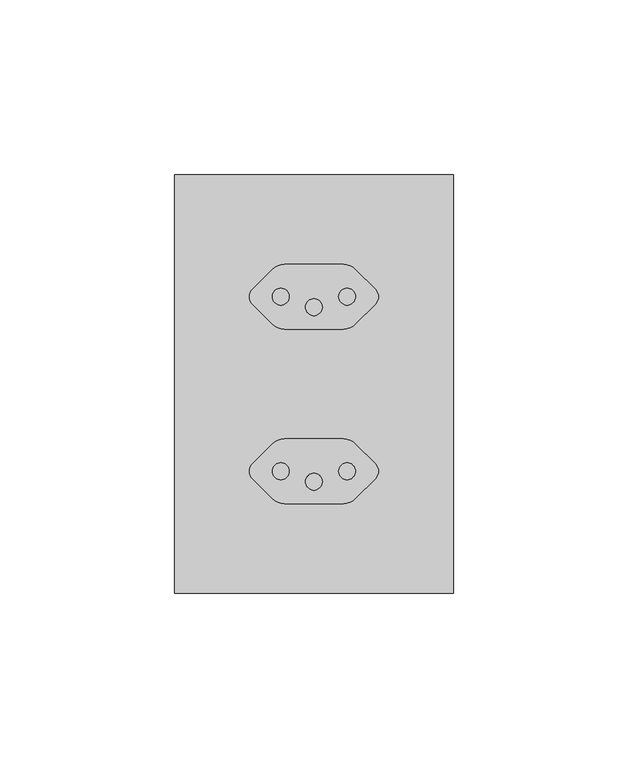
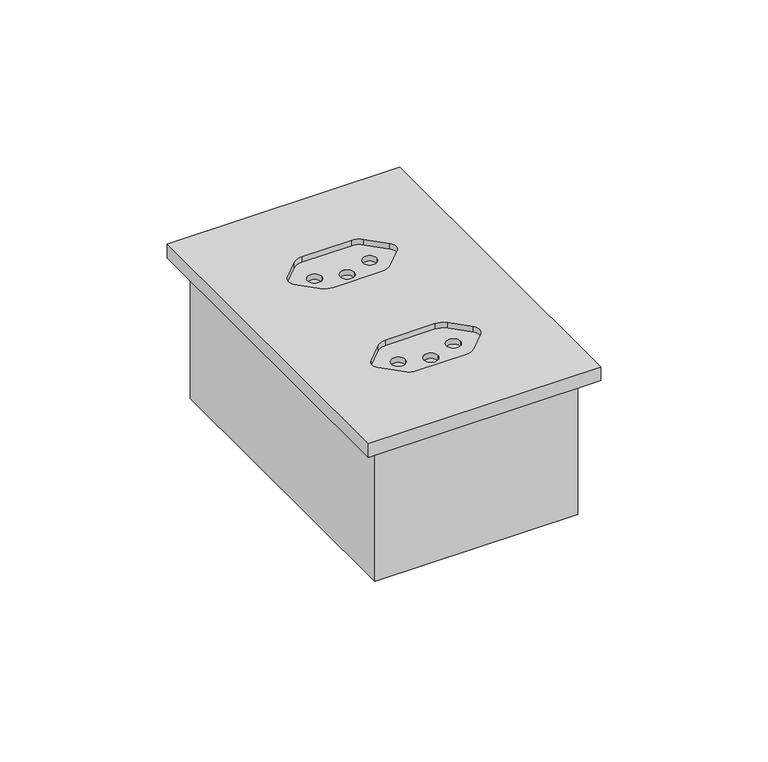
"""IFC4 building model written with IfcOpenShell, lengths in millimetres: proxy geometry, CAIXA VERTICE V7 : Tomada 20A 2s."""

from ifc_helpers import new_model, si_unit, frame, origin, place, context, project, spatial, polyline, circle_curve, faceted_brep, source, transform, mapped, element, save
from ifc_brep_helpers import plane_surface, revolved_surface, advanced_brep


def electrical_fixtures_6b1fb481(model_context):
    return source(origin(), model_context, "Body", "SolidModel", [
        faceted_brep([(33.0, -947.0, -48.0), (-33.0, -947.0, -48.0), (-33.0, -1053.0, -48.0), (33.0, -1053.0, -48.0), (35.0, -1055.0, -50.0), (-35.0, -1055.0, -50.0), (-35.0, -945.0, -50.0), (35.0, -945.0, -50.0), (35.0, -1055.0, 0.0), (-35.0, -1055.0, 0.0), (-35.0, -945.0, 0.0), (35.0, -945.0, 0.0), (33.0, -1053.0, 0.0), (-33.0, -1053.0, 0.0), (-33.0, -947.0, 0.0), (33.0, -947.0, 0.0)], [[[0, 1, 2, 3]], [[4, 5, 6, 7]], [[4, 8, 9, 5]], [[9, 10, 6, 5]], [[10, 11, 7, 6]], [[11, 8, 4, 7]], [[8, 11, 10, 9], [12, 13, 14, 15]], [[15, 0, 3, 12]], [[14, 1, 0, 15]], [[13, 2, 1, 14]], [[12, 3, 2, 13]]]),
        advanced_brep(
        [(40.0, -1060.0, 5.0), (40.0, -940.0, 5.0), (-40.0, -940.0, 5.0), (-40.0, -1060.0, 5.0), (8.4215729, -1015.75, 5.0), (11.9571068, -1017.2144661, 5.0), (17.6213203, -1022.8786797, 5.0), (17.6213203, -1027.1213203, 5.0), (11.9571068, -1032.7855339, 5.0), (8.4215729, -1034.25, 5.0), (-8.4215729, -1034.25, 5.0), (-11.9571068, -1032.7855339, 5.0), (-17.6213203, -1027.1213203, 5.0), (-17.6213203, -1022.8786797, 5.0), (-11.9571068, -1017.2144661, 5.0), (-8.4215729, -1015.75, 5.0), (8.4215729, -965.75, 5.0), (11.9571068, -967.2144661, 5.0), (17.6213203, -972.8786797, 5.0), (17.6213203, -977.1213203, 5.0), (11.9571068, -982.7855339, 5.0), (8.4215729, -984.25, 5.0), (-8.4215729, -984.25, 5.0), (-11.9571068, -982.7855339, 5.0), (-17.6213203, -977.1213203, 5.0), (-17.6213203, -972.8786797, 5.0), (-11.9571068, -967.2144661, 5.0), (-8.4215729, -965.75, 5.0), (-40.0, -1060.0, 0.0), (-40.0, -940.0, 0.0), (40.0, -940.0, 0.0), (40.0, -1060.0, 0.0), (8.4215729, -1015.75, 3.0), (-8.4215729, -1015.75, 3.0), (-11.9571068, -1017.2144661, 3.0), (-17.6213203, -1022.8786797, 3.0), (-17.6213203, -1027.1213203, 3.0), (-11.9571068, -1032.7855339, 3.0), (-8.4215729, -1034.25, 3.0), (8.4215729, -1034.25, 3.0), (11.9571068, -1032.7855339, 3.0), (17.6213203, -1027.1213203, 3.0), (17.6213203, -1022.8786797, 3.0), (11.9571068, -1017.2144661, 3.0), (-7.1, -1025.0, 3.0), (-11.9, -1025.0, 3.0), (11.9, -1025.0, 3.0), (7.1, -1025.0, 3.0), (2.4, -1028.0, 3.0), (-2.4, -1028.0, 3.0), (-11.9, -1025.0, 1.0), (-7.1, -1025.0, 1.0), (7.1, -1025.0, 1.0), (11.9, -1025.0, 1.0), (-2.4, -1028.0, 1.0), (2.4, -1028.0, 1.0), (8.4215729, -965.75, 3.0), (-8.4215729, -965.75, 3.0), (-11.9571068, -967.2144661, 3.0), (-17.6213203, -972.8786797, 3.0), (-17.6213203, -977.1213203, 3.0), (-11.9571068, -982.7855339, 3.0), (-8.4215729, -984.25, 3.0), (8.4215729, -984.25, 3.0), (11.9571068, -982.7855339, 3.0), (17.6213203, -977.1213203, 3.0), (17.6213203, -972.8786797, 3.0), (11.9571068, -967.2144661, 3.0), (-7.1, -975.0, 3.0), (-11.9, -975.0, 3.0), (11.9, -975.0, 3.0), (7.1, -975.0, 3.0), (2.4, -978.0, 3.0), (-2.4, -978.0, 3.0), (-11.9, -975.0, 1.0), (-7.1, -975.0, 1.0), (7.1, -975.0, 1.0), (11.9, -975.0, 1.0), (-2.4, -978.0, 1.0), (2.4, -978.0, 1.0)],
        [
            (0, 1),
            (1, 2),
            (2, 3),
            (3, 0),
            (4, 5, circle_curve(frame((8.4215729, -1020.75, 5.0), z_axis=(0.0, 0.0, -1.0), x_axis=(-1.0, 0.0, 0.0)), 5.0)),
            (5, 6),
            (6, 7, circle_curve(frame((15.5, -1025.0, 5.0), z_axis=(0.0, 0.0, -1.0), x_axis=(-1.0, 0.0, 0.0)), 3.0)),
            (7, 8),
            (8, 9, circle_curve(frame((8.4215729, -1029.25, 5.0), z_axis=(0.0, 0.0, -1.0), x_axis=(-1.0, 0.0, 0.0)), 5.0)),
            (9, 10),
            (10, 11, circle_curve(frame((-8.4215729, -1029.25, 5.0), z_axis=(0.0, 0.0, -1.0), x_axis=(-1.0, 0.0, 0.0)), 5.0)),
            (11, 12),
            (12, 13, circle_curve(frame((-15.5, -1025.0, 5.0), z_axis=(0.0, 0.0, -1.0), x_axis=(-1.0, 0.0, 0.0)), 3.0)),
            (13, 14),
            (14, 15, circle_curve(frame((-8.4215729, -1020.75, 5.0), z_axis=(0.0, 0.0, -1.0), x_axis=(-1.0, 0.0, 0.0)), 5.0)),
            (15, 4),
            (16, 17, circle_curve(frame((8.4215729, -970.75, 5.0), z_axis=(0.0, 0.0, -1.0), x_axis=(-1.0, 0.0, 0.0)), 5.0)),
            (17, 18),
            (18, 19, circle_curve(frame((15.5, -975.0, 5.0), z_axis=(0.0, 0.0, -1.0), x_axis=(-1.0, 0.0, 0.0)), 3.0)),
            (19, 20),
            (20, 21, circle_curve(frame((8.4215729, -979.25, 5.0), z_axis=(0.0, 0.0, -1.0), x_axis=(-1.0, 0.0, 0.0)), 5.0)),
            (21, 22),
            (22, 23, circle_curve(frame((-8.4215729, -979.25, 5.0), z_axis=(0.0, 0.0, -1.0), x_axis=(-1.0, 0.0, 0.0)), 5.0)),
            (23, 24),
            (24, 25, circle_curve(frame((-15.5, -975.0, 5.0), z_axis=(0.0, 0.0, -1.0), x_axis=(-1.0, 0.0, 0.0)), 3.0)),
            (25, 26),
            (26, 27, circle_curve(frame((-8.4215729, -970.75, 5.0), z_axis=(0.0, 0.0, -1.0), x_axis=(-1.0, 0.0, 0.0)), 5.0)),
            (27, 16),
            (28, 29),
            (29, 30),
            (30, 31),
            (31, 28),
            (3, 28),
            (31, 0),
            (2, 29),
            (1, 30),
            (32, 33),
            (33, 34, circle_curve(frame((-8.4215729, -1020.75, 3.0), z_axis=(0.0, 0.0, 1.0), x_axis=(-1.0, 0.0, 0.0)), 5.0)),
            (34, 35),
            (35, 36, circle_curve(frame((-15.5, -1025.0, 3.0), z_axis=(0.0, 0.0, 1.0), x_axis=(-1.0, 0.0, 0.0)), 3.0)),
            (36, 37),
            (37, 38, circle_curve(frame((-8.4215729, -1029.25, 3.0), z_axis=(0.0, 0.0, 1.0), x_axis=(-1.0, 0.0, 0.0)), 5.0)),
            (38, 39),
            (39, 40, circle_curve(frame((8.4215729, -1029.25, 3.0), z_axis=(0.0, 0.0, 1.0), x_axis=(-1.0, 0.0, 0.0)), 5.0)),
            (40, 41),
            (41, 42, circle_curve(frame((15.5, -1025.0, 3.0), z_axis=(0.0, 0.0, 1.0), x_axis=(-1.0, 0.0, 0.0)), 3.0)),
            (42, 43),
            (43, 32, circle_curve(frame((8.4215729, -1020.75, 3.0), z_axis=(0.0, 0.0, 1.0), x_axis=(-1.0, 0.0, 0.0)), 5.0)),
            (44, 45, circle_curve(frame((-9.5, -1025.0, 3.0), z_axis=(0.0, 0.0, -1.0), x_axis=(1.0, -2.301812013077709e-12, 0.0)), 2.4)),
            (45, 44, circle_curve(frame((-9.5, -1025.0, 3.0), z_axis=(0.0, 0.0, -1.0), x_axis=(1.0, -2.301812013077709e-12, 0.0)), 2.4)),
            (46, 47, circle_curve(frame((9.5, -1025.0, 3.0), z_axis=(0.0, 0.0, -1.0), x_axis=(1.0, -2.301812013077709e-12, 0.0)), 2.4)),
            (47, 46, circle_curve(frame((9.5, -1025.0, 3.0), z_axis=(0.0, 0.0, -1.0), x_axis=(1.0, -2.301812013077709e-12, 0.0)), 2.4)),
            (48, 49, circle_curve(frame((0.0, -1028.0, 3.0), z_axis=(0.0, 0.0, -1.0), x_axis=(1.0, -2.301812013077709e-12, 0.0)), 2.4)),
            (49, 48, circle_curve(frame((0.0, -1028.0, 3.0), z_axis=(0.0, 0.0, -1.0), x_axis=(1.0, -2.301812013077709e-12, 0.0)), 2.4)),
            (32, 4),
            (15, 33),
            (14, 34),
            (13, 35),
            (12, 36),
            (11, 37),
            (10, 38),
            (9, 39),
            (8, 40),
            (7, 41),
            (6, 42),
            (5, 43),
            (50, 51, circle_curve(frame((-9.5, -1025.0, 1.0), z_axis=(0.0, 0.0, 1.0), x_axis=(1.0, -2.301812013077709e-12, 0.0)), 2.4)),
            (51, 50, circle_curve(frame((-9.5, -1025.0, 1.0), z_axis=(0.0, 0.0, 1.0), x_axis=(1.0, -2.301812013077709e-12, 0.0)), 2.4)),
            (52, 53, circle_curve(frame((9.5, -1025.0, 1.0), z_axis=(0.0, 0.0, 1.0), x_axis=(1.0, -2.301812013077709e-12, 0.0)), 2.4)),
            (53, 52, circle_curve(frame((9.5, -1025.0, 1.0), z_axis=(0.0, 0.0, 1.0), x_axis=(1.0, -2.301812013077709e-12, 0.0)), 2.4)),
            (54, 55, circle_curve(frame((0.0, -1028.0, 1.0), z_axis=(0.0, 0.0, 1.0), x_axis=(1.0, -2.301812013077709e-12, 0.0)), 2.4)),
            (55, 54, circle_curve(frame((0.0, -1028.0, 1.0), z_axis=(0.0, 0.0, 1.0), x_axis=(1.0, -2.301812013077709e-12, 0.0)), 2.4)),
            (45, 50),
            (51, 44),
            (47, 52),
            (53, 46),
            (49, 54),
            (55, 48),
            (56, 57),
            (57, 58, circle_curve(frame((-8.4215729, -970.75, 3.0), z_axis=(0.0, 0.0, 1.0), x_axis=(-1.0, 0.0, 0.0)), 5.0)),
            (58, 59),
            (59, 60, circle_curve(frame((-15.5, -975.0, 3.0), z_axis=(0.0, 0.0, 1.0), x_axis=(-1.0, 0.0, 0.0)), 3.0)),
            (60, 61),
            (61, 62, circle_curve(frame((-8.4215729, -979.25, 3.0), z_axis=(0.0, 0.0, 1.0), x_axis=(-1.0, 0.0, 0.0)), 5.0)),
            (62, 63),
            (63, 64, circle_curve(frame((8.4215729, -979.25, 3.0), z_axis=(0.0, 0.0, 1.0), x_axis=(-1.0, 0.0, 0.0)), 5.0)),
            (64, 65),
            (65, 66, circle_curve(frame((15.5, -975.0, 3.0), z_axis=(0.0, 0.0, 1.0), x_axis=(-1.0, 0.0, 0.0)), 3.0)),
            (66, 67),
            (67, 56, circle_curve(frame((8.4215729, -970.75, 3.0), z_axis=(0.0, 0.0, 1.0), x_axis=(-1.0, 0.0, 0.0)), 5.0)),
            (68, 69, circle_curve(frame((-9.5, -975.0, 3.0), z_axis=(0.0, 0.0, -1.0), x_axis=(1.0, -2.301812013077709e-12, 0.0)), 2.4)),
            (69, 68, circle_curve(frame((-9.5, -975.0, 3.0), z_axis=(0.0, 0.0, -1.0), x_axis=(1.0, -2.301812013077709e-12, 0.0)), 2.4)),
            (70, 71, circle_curve(frame((9.5, -975.0, 3.0), z_axis=(0.0, 0.0, -1.0), x_axis=(1.0, -2.301812013077709e-12, 0.0)), 2.4)),
            (71, 70, circle_curve(frame((9.5, -975.0, 3.0), z_axis=(0.0, 0.0, -1.0), x_axis=(1.0, -2.301812013077709e-12, 0.0)), 2.4)),
            (72, 73, circle_curve(frame((0.0, -978.0, 3.0), z_axis=(0.0, 0.0, -1.0), x_axis=(1.0, -2.301812013077709e-12, 0.0)), 2.4)),
            (73, 72, circle_curve(frame((0.0, -978.0, 3.0), z_axis=(0.0, 0.0, -1.0), x_axis=(1.0, -2.301812013077709e-12, 0.0)), 2.4)),
            (56, 16),
            (27, 57),
            (26, 58),
            (25, 59),
            (24, 60),
            (23, 61),
            (22, 62),
            (21, 63),
            (20, 64),
            (19, 65),
            (18, 66),
            (17, 67),
            (74, 75, circle_curve(frame((-9.5, -975.0, 1.0), z_axis=(0.0, 0.0, 1.0), x_axis=(1.0, -2.301812013077709e-12, 0.0)), 2.4)),
            (75, 74, circle_curve(frame((-9.5, -975.0, 1.0), z_axis=(0.0, 0.0, 1.0), x_axis=(1.0, -2.301812013077709e-12, 0.0)), 2.4)),
            (76, 77, circle_curve(frame((9.5, -975.0, 1.0), z_axis=(0.0, 0.0, 1.0), x_axis=(1.0, -2.301812013077709e-12, 0.0)), 2.4)),
            (77, 76, circle_curve(frame((9.5, -975.0, 1.0), z_axis=(0.0, 0.0, 1.0), x_axis=(1.0, -2.301812013077709e-12, 0.0)), 2.4)),
            (78, 79, circle_curve(frame((0.0, -978.0, 1.0), z_axis=(0.0, 0.0, 1.0), x_axis=(1.0, -2.301812013077709e-12, 0.0)), 2.4)),
            (79, 78, circle_curve(frame((0.0, -978.0, 1.0), z_axis=(0.0, 0.0, 1.0), x_axis=(1.0, -2.301812013077709e-12, 0.0)), 2.4)),
            (69, 74),
            (75, 68),
            (71, 76),
            (77, 70),
            (73, 78),
            (79, 72),
        ],
        [
            plane_surface(frame((-60.0, -1060.0, 5.0), z_axis=(0.0, 0.0, 1.0), x_axis=(-1.0, 0.0, 0.0))),
            plane_surface(frame((-60.0, -1060.0, 0.0), z_axis=(0.0, 0.0, -1.0), x_axis=(1.0, 0.0, 0.0))),
            plane_surface(frame((40.0, -1060.0, 5.0), z_axis=(0.0, -1.0, 0.0), x_axis=(0.0, 0.0, -1.0))),
            plane_surface(frame((-40.0, -1060.0, 5.0), z_axis=(-1.0, 0.0, 0.0), x_axis=(0.0, 0.0, -1.0))),
            plane_surface(frame((-40.0, -940.0, 5.0), z_axis=(0.0, 1.0, 0.0), x_axis=(0.0, 0.0, -1.0))),
            plane_surface(frame((40.0, -940.0, 5.0), z_axis=(1.0, 0.0, 0.0), x_axis=(0.0, 0.0, -1.0))),
            plane_surface(frame((3.4215729, -1020.75, 3.0), z_axis=(0.0, 0.0, 1.0), x_axis=(0.0, -1.0, 0.0))),
            plane_surface(frame((-8.4215729, -1015.75, 5.0), z_axis=(0.0, -1.0, 0.0), x_axis=(0.0, 0.0, -1.0))),
            revolved_surface(polyline([(-13.4215729, -1020.75, 5.0), (-13.4215729, -1020.75, 3.0)]), (-8.4215729, -1020.75, 3.0), (0.0, 0.0, 1.0)),
            plane_surface(frame((-17.6213203, -1022.8786797, 5.0), z_axis=(0.7071067811865045, -0.7071067811865905, 0.0), x_axis=(0.0, 0.0, -1.0))),
            revolved_surface(polyline([(-18.5, -1025.0, 5.0), (-18.5, -1025.0, 3.0)]), (-15.5, -1025.0, 3.0), (0.0, 0.0, 1.0)),
            plane_surface(frame((-11.9571068, -1032.7855339, 5.0), z_axis=(0.7071067811865515, 0.7071067811865437, 0.0), x_axis=(0.0, 0.0, -1.0))),
            revolved_surface(polyline([(-13.4215729, -1029.25, 5.0), (-13.4215729, -1029.25, 3.0)]), (-8.4215729, -1029.25, 3.0), (0.0, 0.0, 1.0)),
            plane_surface(frame((8.4215729, -1034.25, 5.0), z_axis=(0.0, 1.0, 0.0), x_axis=(0.0, 0.0, -1.0))),
            revolved_surface(polyline([(3.4215728999999993, -1029.25, 5.0), (3.4215728999999993, -1029.25, 3.0)]), (8.4215729, -1029.25, 3.0), (0.0, 0.0, 1.0)),
            plane_surface(frame((17.6213203, -1027.1213203, 5.0), z_axis=(-0.7071067811865307, 0.7071067811865643, 0.0), x_axis=(0.0, 0.0, -1.0))),
            revolved_surface(polyline([(12.5, -1025.0, 5.0), (12.5, -1025.0, 3.0)]), (15.5, -1025.0, 3.0), (0.0, 0.0, 1.0)),
            plane_surface(frame((11.9571068, -1017.2144661, 5.0), z_axis=(-0.7071067811865893, -0.7071067811865058, 0.0), x_axis=(0.0, 0.0, -1.0))),
            revolved_surface(polyline([(3.4215728999999993, -1020.75, 5.0), (3.4215728999999993, -1020.75, 3.0)]), (8.4215729, -1020.75, 3.0), (0.0, 0.0, 1.0)),
            plane_surface(frame((-7.1, -1025.0, 1.0), z_axis=(0.0, 0.0, 1.0), x_axis=(2.301812013077709e-12, 1.0, 0.0))),
            revolved_surface(polyline([(-7.1, -1025.0000000000055, 3.0), (-7.1, -1025.0000000000055, 1.0)]), (-9.5, -1025.0, 1.0), (0.0, 0.0, 1.0)),
            revolved_surface(polyline([(11.9, -1025.0000000000055, 3.0), (11.9, -1025.0000000000055, 1.0)]), (9.5, -1025.0, 5.0), (0.0, 0.0, 1.0)),
            revolved_surface(polyline([(2.4, -1028.0000000000055, 3.0), (2.4, -1028.0000000000055, 1.0)]), (0.0, -1028.0, 5.0), (0.0, 0.0, 1.0)),
            plane_surface(frame((3.4215729, -970.75, 3.0), z_axis=(0.0, 0.0, 1.0), x_axis=(0.0, -1.0, 0.0))),
            plane_surface(frame((-8.4215729, -965.75, 5.0), z_axis=(0.0, -1.0, 0.0), x_axis=(0.0, 0.0, -1.0))),
            revolved_surface(polyline([(-13.4215729, -970.75, 5.0), (-13.4215729, -970.75, 3.0)]), (-8.4215729, -970.75, 3.0), (0.0, 0.0, 1.0)),
            plane_surface(frame((-17.6213203, -972.8786797, 5.0), z_axis=(0.7071067811865045, -0.7071067811865905, 0.0), x_axis=(0.0, 0.0, -1.0))),
            revolved_surface(polyline([(-18.5, -975.0, 5.0), (-18.5, -975.0, 3.0)]), (-15.5, -975.0, 3.0), (0.0, 0.0, 1.0)),
            plane_surface(frame((-11.9571068, -982.7855339, 5.0), z_axis=(0.7071067811865515, 0.7071067811865437, 0.0), x_axis=(0.0, 0.0, -1.0))),
            revolved_surface(polyline([(-13.4215729, -979.25, 5.0), (-13.4215729, -979.25, 3.0)]), (-8.4215729, -979.25, 3.0), (0.0, 0.0, 1.0)),
            plane_surface(frame((8.4215729, -984.25, 5.0), z_axis=(0.0, 1.0, 0.0), x_axis=(0.0, 0.0, -1.0))),
            revolved_surface(polyline([(3.4215728999999993, -979.25, 5.0), (3.4215728999999993, -979.25, 3.0)]), (8.4215729, -979.25, 3.0), (0.0, 0.0, 1.0)),
            plane_surface(frame((17.6213203, -977.1213203, 5.0), z_axis=(-0.7071067811865307, 0.7071067811865643, 0.0), x_axis=(0.0, 0.0, -1.0))),
            revolved_surface(polyline([(12.5, -975.0, 5.0), (12.5, -975.0, 3.0)]), (15.5, -975.0, 3.0), (0.0, 0.0, 1.0)),
            plane_surface(frame((11.9571068, -967.2144661, 5.0), z_axis=(-0.7071067811865893, -0.7071067811865058, 0.0), x_axis=(0.0, 0.0, -1.0))),
            revolved_surface(polyline([(3.4215728999999993, -970.75, 5.0), (3.4215728999999993, -970.75, 3.0)]), (8.4215729, -970.75, 3.0), (0.0, 0.0, 1.0)),
            plane_surface(frame((-7.1, -975.0, 1.0), z_axis=(0.0, 0.0, 1.0), x_axis=(2.301812013077709e-12, 1.0, 0.0))),
            revolved_surface(polyline([(-7.1, -975.0000000000056, 3.0), (-7.1, -975.0000000000056, 1.0)]), (-9.5, -975.0, 1.0), (0.0, 0.0, 1.0)),
            revolved_surface(polyline([(11.9, -975.0000000000056, 3.0), (11.9, -975.0000000000056, 1.0)]), (9.5, -975.0, 5.0), (0.0, 0.0, 1.0)),
            revolved_surface(polyline([(2.4, -978.0000000000056, 3.0), (2.4, -978.0000000000056, 1.0)]), (0.0, -978.0, 5.0), (0.0, 0.0, 1.0)),
        ],
        [
            (0, [[1, 2, 3, 4], [5, 6, 7, 8, 9, 10, 11, 12, 13, 14, 15, 16], [17, 18, 19, 20, 21, 22, 23, 24, 25, 26, 27, 28]]),
            (1, [[29, 30, 31, 32]]),
            (2, [[33, -32, 34, -4]]),
            (3, [[35, -29, -33, -3]]),
            (4, [[36, -30, -35, -2]]),
            (5, [[-34, -31, -36, -1]]),
            (6, [[37, 38, 39, 40, 41, 42, 43, 44, 45, 46, 47, 48], [49, 50], [51, 52], [53, 54]]),
            (7, [[55, -16, 56, -37]]),
            (8, [[-56, -15, 57, -38]]),
            (9, [[-57, -14, 58, -39]]),
            (10, [[-58, -13, 59, -40]]),
            (11, [[-59, -12, 60, -41]]),
            (12, [[-60, -11, 61, -42]]),
            (13, [[-61, -10, 62, -43]]),
            (14, [[-62, -9, 63, -44]]),
            (15, [[-63, -8, 64, -45]]),
            (16, [[-64, -7, 65, -46]]),
            (17, [[-65, -6, 66, -47]]),
            (18, [[-66, -5, -55, -48]]),
            (19, [[67, 68]]),
            (19, [[69, 70]]),
            (19, [[71, 72]]),
            (20, [[73, -68, 74, -50]]),
            (20, [[-74, -67, -73, -49]]),
            (21, [[75, -70, 76, -52]]),
            (21, [[-76, -69, -75, -51]]),
            (22, [[77, -72, 78, -54]]),
            (22, [[-78, -71, -77, -53]]),
            (23, [[79, 80, 81, 82, 83, 84, 85, 86, 87, 88, 89, 90], [91, 92], [93, 94], [95, 96]]),
            (24, [[97, -28, 98, -79]]),
            (25, [[-98, -27, 99, -80]]),
            (26, [[-99, -26, 100, -81]]),
            (27, [[-100, -25, 101, -82]]),
            (28, [[-101, -24, 102, -83]]),
            (29, [[-102, -23, 103, -84]]),
            (30, [[-103, -22, 104, -85]]),
            (31, [[-104, -21, 105, -86]]),
            (32, [[-105, -20, 106, -87]]),
            (33, [[-106, -19, 107, -88]]),
            (34, [[-107, -18, 108, -89]]),
            (35, [[-108, -17, -97, -90]]),
            (36, [[109, 110]]),
            (36, [[111, 112]]),
            (36, [[113, 114]]),
            (37, [[115, -110, 116, -92]]),
            (37, [[-116, -109, -115, -91]]),
            (38, [[117, -112, 118, -94]]),
            (38, [[-118, -111, -117, -93]]),
            (39, [[119, -114, 120, -96]]),
            (39, [[-120, -113, -119, -95]]),
        ],
    ),
    ])


if __name__ == "__main__":
    model = new_model("IFC4")
    model_context = context("Model", 3, world=origin())
    ifc_project = project(units=[si_unit("LENGTHUNIT", "METRE", prefix="MILLI")], contexts=[model_context])
    site = spatial("IfcSite", under=ifc_project)
    building = spatial("IfcBuilding", under=site)
    placement = place(None, origin())
    electrical_fixtures_shape = electrical_fixtures_6b1fb481(model_context)
    element("IfcBuildingElementProxy", 1, Name="CAIXA VERTICE V7 : Tomada 20A 2s", ObjectType="CAIXA VERTICE V7 : Tomada 20A 2s", at=placement, inside=building, context=model_context, shape_type="MappedRepresentation", body=[
        mapped(electrical_fixtures_shape, transform((0.0, 0.0, 0.0), x_axis=(1.0, 0.0, 0.0), y_axis=(0.0, 1.0, 0.0), z_axis=(0.0, 0.0, 1.0))),
    ])
    save(model, "model.ifc")

# Revit data of these elements
# Type "CAIXA VERTICE V7 : Tomada 20A 2s"
#   URL = "www.facebook.com/verticetreinamentos"
#   SEÇÃO [instance default] = ""
#   Rotação [instance default] = 0.00°
#   LARGURA DA TAMPA = 0.08 m
#   BORDA = 0.01 m
#   ALTURA DE INSTALAÇÃO [instance default] = 1.10 m
#   Distância Anotação [instance default] = 0.0015 m
#   ALTURA DA TAMPA = 0.12 m
#   Vertical [instance default] = yes
#   VER SEÇÃO [instance default] = no
#   SHADE ESQ [instance default] = no
#   SHADE DIR [instance default] = yes
#   HORIZONTAL [instance default] = no
#   ANDAR COM A LEGENDA [instance default] = 0
#   Material Tampa [instance default] = Plástico, branco opaco
#   Caixa = element 1798518
#   Anotação = element 1798532
#   Default Elevation = 0
# Element 1 (IfcBuildingElementProxy, "CAIXA VERTICE V7 : Tomada 20A 2s")
#   ALTURA DE INSTALAÇÃO = 1.00 m
#   Materials on its faces: "Plástico, branco opaco"
# Materials
#   "Plástico, branco opaco": class "Plástico", colour RGB 120 120 120, transparency 0, Description = "Plastic, generic, opaque white", Cost = 0
